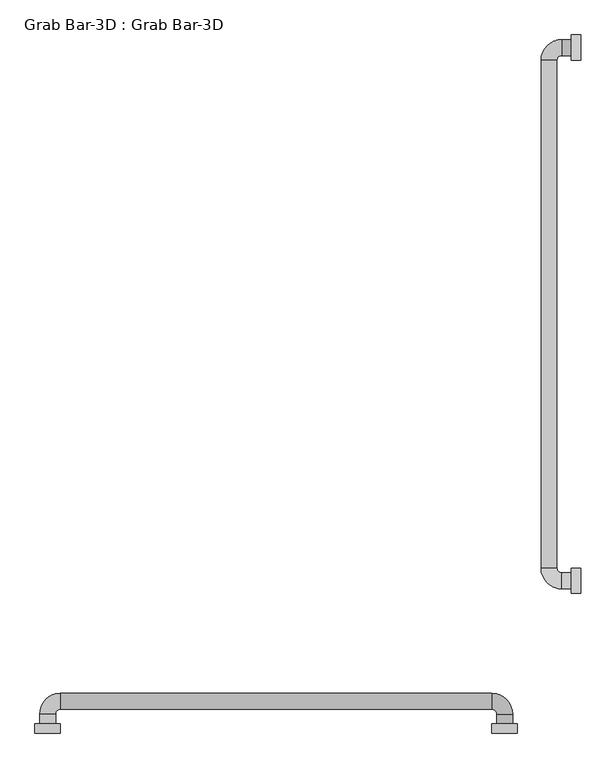
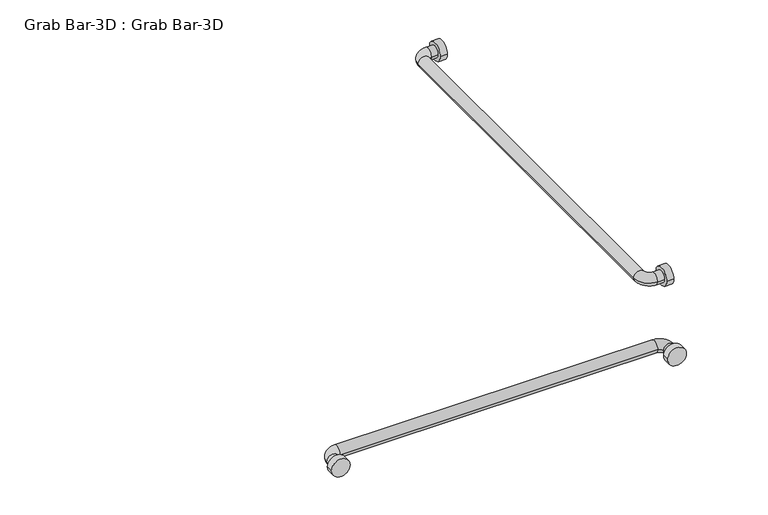
"""IFC4 building model written with IfcOpenShell, lengths in millimetres: proxy geometry, Grab Bar-3D : Grab Bar-3D."""

import ifcopenshell
import ifcopenshell.guid

model = None  # the IFC model being written
_history = None  # IfcOwnerHistory: only IFC2X3 demands one
_inside = {}  # id of a spatial element -> (the spatial element, [elements in it])
_under = {}  # id of a project, library or spatial element -> (it, [spatial elements below it])
_declared = {}  # id of a project -> (the project, [libraries it declares])
_typed = {}  # id of a type object -> (the type object, [elements of that type])
_made_of = {}  # id of a material, layer set ... -> (it, [elements and type objects made of it])


def new_model(schema):
    """Start an empty IFC model of exactly this schema.

    Asked for "IFC4X3", IfcOpenShell would pick the latest addendum, in which some entities
    have other attributes; the version numbers below select the first issue.
    IFC2X3 requires an IfcOwnerHistory on every rooted entity: one is made here for all.
    """
    global model, _history
    if schema == "IFC4X3":
        model = ifcopenshell.file(schema_version=(4, 3, 0, 0))
    else:
        model = ifcopenshell.file(schema=schema)
    _inside.clear()
    _under.clear()
    _declared.clear()
    _typed.clear()
    _made_of.clear()
    _history = None
    if model.schema == "IFC2X3":
        org = make("IfcOrganization", Name="unknown")
        user = make(
            "IfcPersonAndOrganization",
            ThePerson=make("IfcPerson", FamilyName="unknown"),
            TheOrganization=org,
        )
        app = make(
            "IfcApplication",
            ApplicationDeveloper=org,
            Version="unknown",
            ApplicationFullName="unknown",
            ApplicationIdentifier="unknown",
        )
        _history = make(
            "IfcOwnerHistory",
            OwningUser=user,
            OwningApplication=app,
            ChangeAction="ADDED",
            CreationDate=0,
        )
    return model


def make(cls, **values):
    """One entity of the class cls with the attributes given. An attribute that is None is left unset."""
    return model.create_entity(
        cls, **{name: value for name, value in values.items() if value is not None}
    )


def rooted(cls, **values):
    """An entity with a GlobalId (a new one), such as an element, a storey or a relation."""
    return make(cls, GlobalId=ifcopenshell.guid.new(), OwnerHistory=_history, **values)


def si_unit(unit_type, name, prefix=None):
    """IfcSIUnit, for example si_unit("LENGTHUNIT", "METRE", prefix="MILLI")."""
    return make("IfcSIUnit", UnitType=unit_type, Prefix=prefix, Name=name)


def assignment(units):
    """IfcUnitAssignment: the units of a project."""
    return None if units is None else make("IfcUnitAssignment", Units=units)


def point(xyz):
    """IfcCartesianPoint."""
    return None if xyz is None else make("IfcCartesianPoint", Coordinates=xyz)


def direction(xyz):
    """IfcDirection."""
    return None if xyz is None else make("IfcDirection", DirectionRatios=xyz)


def frame(location, z_axis=None, x_axis=None):
    """IfcAxis2Placement3D, a coordinate frame: its origin and axes. An axis left out is left unset."""
    return make(
        "IfcAxis2Placement3D",
        Location=point(location),
        Axis=direction(z_axis),
        RefDirection=direction(x_axis),
    )


def frame_2d(location, x_axis=None):
    """IfcAxis2Placement2D, a coordinate frame in the plane: its origin and x axis."""
    return make(
        "IfcAxis2Placement2D", Location=point(location), RefDirection=direction(x_axis)
    )


def origin():
    """The frame at (0, 0, 0) with its axes left unset."""
    return frame((0.0, 0.0, 0.0))


def place(relative_to, where):
    """IfcLocalPlacement: puts the frame where relative to a parent placement (None: the world)."""
    return make(
        "IfcLocalPlacement", PlacementRelTo=relative_to, RelativePlacement=where
    )


def context(
    kind, dimensions, precision=None, world=None, true_north=None, identifier=None
):
    """IfcGeometricRepresentationContext, for example the 3D "Model" context."""
    return make(
        "IfcGeometricRepresentationContext",
        ContextIdentifier=identifier,
        ContextType=kind,
        CoordinateSpaceDimension=dimensions,
        Precision=precision,
        WorldCoordinateSystem=world,
        TrueNorth=true_north,
    )


def project(units=None, contexts=None):
    """IfcProject with its units and contexts."""
    return rooted(
        "IfcProject",
        Name="project",
        RepresentationContexts=contexts,
        UnitsInContext=assignment(units),
    )


def spatial(cls, under=None, at=None, **own):
    """A site, building, storey or space (cls), placed at a placement, below another one or the project."""
    s = rooted(cls, ObjectPlacement=at, **own)
    if under is not None:
        _under.setdefault(under.id(), (under, []))[1].append(s)
    return s


def circle_curve(where, radius):
    """IfcCircle in the frame where."""
    return make("IfcCircle", Position=where, Radius=radius)


def ellipse_curve(where, semi_axis1, semi_axis2):
    """IfcEllipse in the frame where."""
    return make(
        "IfcEllipse", Position=where, SemiAxis1=semi_axis1, SemiAxis2=semi_axis2
    )


def trimmed(basis, trim1, trim2, sense, master):
    """IfcTrimmedCurve: the piece of a basis curve between two trims."""
    return make(
        "IfcTrimmedCurve",
        BasisCurve=basis,
        Trim1=trim1,
        Trim2=trim2,
        SenseAgreement=sense,
        MasterRepresentation=master,
    )


def segment(curve, same_sense, transition):
    """IfcCompositeCurveSegment."""
    return make(
        "IfcCompositeCurveSegment",
        Transition=transition,
        SameSense=same_sense,
        ParentCurve=curve,
    )


def composite_curve(segments, self_intersect=None):
    """IfcCompositeCurve: segments joined end to end."""
    return make("IfcCompositeCurve", Segments=segments, SelfIntersect=self_intersect)


def outline(outer, holes=None, kind="AREA"):
    """IfcArbitraryClosedProfileDef: a profile drawn as a closed curve; with holes, ...WithVoids."""
    if holes is None:
        return make("IfcArbitraryClosedProfileDef", ProfileType=kind, OuterCurve=outer)
    return make(
        "IfcArbitraryProfileDefWithVoids",
        ProfileType=kind,
        OuterCurve=outer,
        InnerCurves=holes,
    )


def extrude(swept, where, along, depth):
    """IfcExtrudedAreaSolid: the profile swept, set in the frame where, extruded along a direction by depth."""
    return make(
        "IfcExtrudedAreaSolid",
        SweptArea=swept,
        Position=where,
        ExtrudedDirection=direction(along),
        Depth=depth,
    )


def shape(context_of_items, identifier, shape_type, items):
    """IfcShapeRepresentation: the items that make up one representation, for example the "Body"."""
    return make(
        "IfcShapeRepresentation",
        ContextOfItems=context_of_items,
        RepresentationIdentifier=identifier,
        RepresentationType=shape_type,
        Items=items,
    )


def source(mapping_origin, context_of_items, identifier, shape_type, items):
    """IfcRepresentationMap: a shape defined once, which mapped items show again and again."""
    return make(
        "IfcRepresentationMap",
        MappingOrigin=mapping_origin,
        MappedRepresentation=shape(context_of_items, identifier, shape_type, items),
    )


def transform(
    local_origin,
    x_axis=None,
    y_axis=None,
    z_axis=None,
    scale=None,
    scale2=None,
    scale3=None,
    uniform=True,
):
    """IfcCartesianTransformationOperator3D, or its non-uniform kind. x_axis, y_axis, z_axis: its Axis1, 2, 3."""
    if uniform:
        return make(
            "IfcCartesianTransformationOperator3D",
            Axis1=direction(x_axis),
            Axis2=direction(y_axis),
            LocalOrigin=point(local_origin),
            Scale=scale,
            Axis3=direction(z_axis),
        )
    return make(
        "IfcCartesianTransformationOperator3DnonUniform",
        Axis1=direction(x_axis),
        Axis2=direction(y_axis),
        LocalOrigin=point(local_origin),
        Scale=scale,
        Axis3=direction(z_axis),
        Scale2=scale2,
        Scale3=scale3,
    )


def mapped(mapping_source, mapping_target):
    """IfcMappedItem: shows the shape of a source again, moved by a transform."""
    return make(
        "IfcMappedItem", MappingSource=mapping_source, MappingTarget=mapping_target
    )


def made_of(thing, what):
    """Note that an element or type object is made of a material, layer set ...; save() writes the relation."""
    if what is not None:
        _made_of.setdefault(what.id(), (what, []))[1].append(thing)
    return thing


def element(
    cls,
    number,
    at=None,
    inside=None,
    cuts=None,
    type_object=None,
    material=None,
    context=None,
    identifier="Body",
    shape_type=None,
    held_by="IfcProductDefinitionShape",
    body=None,
    shapes=None,
    **own,
):
    """One element of the class cls, such as IfcWall. Its Tag is "e" and its number.

    at: its placement. inside: the storey or other place that contains it. cuts: it is an
    opening in that element (IfcRelVoidsElement). A single representation is given by context,
    identifier, shape_type and body (its items); several are given by shapes. held_by: the class
    of the entity that holds the representations. save() writes the other relations.
    """
    e = rooted(cls, Tag="e%d" % number, ObjectPlacement=at, **own)
    if body is not None:
        shapes = [shape(context, identifier, shape_type, body)]
    if shapes is not None:
        e.Representation = make(held_by, Representations=shapes)
    if inside is not None:
        _inside.setdefault(inside.id(), (inside, []))[1].append(e)
    if cuts is not None:
        rooted(
            "IfcRelVoidsElement", RelatingBuildingElement=cuts, RelatedOpeningElement=e
        )
    if type_object is not None:
        _typed.setdefault(type_object.id(), (type_object, []))[1].append(e)
    return made_of(e, material)


def aggregate(whole, parts):
    """IfcRelAggregates: a whole, such as a stair, and the parts it consists of."""
    return rooted("IfcRelAggregates", RelatingObject=whole, RelatedObjects=parts)


def save(model, path):
    """Write the relations noted so far, then the file.

    IfcRelAggregates (storeys below a building ...), IfcRelContainedInSpatialStructure (elements
    in a storey), IfcRelDefinesByType, IfcRelAssociatesMaterial and IfcRelDeclares: one each for
    every whole, place, type object, material and project.
    """
    for whole, parts in _under.values():
        aggregate(whole, parts)
    for where, things in _inside.values():
        rooted(
            "IfcRelContainedInSpatialStructure",
            RelatedElements=things,
            RelatingStructure=where,
        )
    for kind, things in _typed.values():
        rooted("IfcRelDefinesByType", RelatedObjects=things, RelatingType=kind)
    for what, things in _made_of.values():
        rooted("IfcRelAssociatesMaterial", RelatedObjects=things, RelatingMaterial=what)
    for by, libraries in _declared.values():
        rooted("IfcRelDeclares", RelatingContext=by, RelatedDefinitions=libraries)
    model.write(path)


def plane_surface(at):
    """IfcPlane: the flat surface through the origin of the frame at, square to its z axis."""
    return make("IfcPlane", Position=at)


def cylinder_surface(at, radius):
    """IfcCylindricalSurface: all points at the distance radius from the z axis of the frame at."""
    return make("IfcCylindricalSurface", Position=at, Radius=radius)


def revolved_surface(curve, axis_point, axis_direction):
    """IfcSurfaceOfRevolution: the curve turned about the line through axis_point along axis_direction."""
    return make(
        "IfcSurfaceOfRevolution",
        SweptCurve=make("IfcArbitraryOpenProfileDef", ProfileType="CURVE", Curve=curve),
        AxisPosition=make("IfcAxis1Placement", Location=point(axis_point), Axis=direction(axis_direction)),
    )


def advanced_brep(points, edges, surfaces, faces):
    """IfcAdvancedBrep: a solid bounded by faces that lie on surfaces and meet in shared edges.

    An edge is (start, end): straight between two places in points (the first is 0);
    or (start, end, curve); or (start, end, curve, False) where it runs against its curve.
    A face is (place in surfaces, loops), or (place, loops, False) where it looks against
    its surface's normal. A loop lists edges by number (the first is 1), with a minus sign
    where the edge is run from its end to its start. The first loop is the outer one.
    """
    corners = [point(p) for p in points]
    vertices = [make("IfcVertexPoint", VertexGeometry=c) for c in corners]
    made = []
    for start, end, *more in edges:
        made.append(
            make(
                "IfcEdgeCurve",
                EdgeStart=vertices[start],
                EdgeEnd=vertices[end],
                EdgeGeometry=more[0] if more else make("IfcPolyline", Points=[corners[start], corners[end]]),
                SameSense=more[1] if len(more) > 1 else True,
            )
        )
    hull = []
    for where, loops, *sense in faces:
        bounds = []
        for j, loop in enumerate(loops):
            ring = [make("IfcOrientedEdge", EdgeElement=made[abs(k) - 1], Orientation=k > 0) for k in loop]
            bounds.append(
                make(
                    "IfcFaceOuterBound" if j == 0 else "IfcFaceBound",
                    Bound=make("IfcEdgeLoop", EdgeList=ring),
                    Orientation=True,
                )
            )
        hull.append(make("IfcAdvancedFace", Bounds=bounds, FaceSurface=surfaces[where], SameSense=sense[0] if sense else True))
    return make("IfcAdvancedBrep", Outer=make("IfcClosedShell", CfsFaces=hull))


def grab_bar_3d_grab_bar_3d_00f4341b(model_context):
    return source(origin(), model_context, "Body", "SolidModel", [
        extrude(outline(composite_curve([segment(trimmed(circle_curve(frame_2d((304.8, 914.4)), 25.4), [point((279.4, 914.4))], [point((330.2, 914.4))], False, "CARTESIAN"), True, "CONTINUOUS"), segment(trimmed(circle_curve(frame_2d((304.8, 914.4)), 25.4), [point((330.2, 914.4))], [point((279.4, 914.4))], False, "CARTESIAN"), True, "CONTINUOUS")], self_intersect=False)), frame((-19.05, 0.0, 0.0), z_axis=(1.0, 0.0, 0.0), x_axis=(0.0, 1.0, 0.0)), (0.0, 0.0, 1.0), 19.05),
        extrude(outline(composite_curve([segment(trimmed(circle_curve(frame_2d((1371.6, 914.4)), 25.4), [point((1346.2, 914.4))], [point((1397.0, 914.4))], False, "CARTESIAN"), True, "CONTINUOUS"), segment(trimmed(circle_curve(frame_2d((1371.6, 914.4)), 25.4), [point((1397.0, 914.4))], [point((1346.2, 914.4))], False, "CARTESIAN"), True, "CONTINUOUS")], self_intersect=False)), frame((-19.05, 0.0, 0.0), z_axis=(1.0, 0.0, 0.0), x_axis=(0.0, 1.0, 0.0)), (0.0, 0.0, 1.0), 19.05),
        extrude(outline(composite_curve([segment(trimmed(circle_curve(frame_2d((914.4, -152.4)), 25.4), [point((914.4, -177.8))], [point((914.4, -127.0))], False, "CARTESIAN"), True, "CONTINUOUS"), segment(trimmed(circle_curve(frame_2d((914.4, -152.4)), 25.4), [point((914.4, -127.0))], [point((914.4, -177.8))], False, "CARTESIAN"), True, "CONTINUOUS")], self_intersect=False)), frame((0.0, 0.0, 0.0), z_axis=(0.0, 1.0, 0.0), x_axis=(0.0, 0.0, 1.0)), (0.0, 0.0, 1.0), 19.05),
        extrude(outline(composite_curve([segment(trimmed(circle_curve(frame_2d((914.4, -1066.8)), 25.4), [point((914.4, -1092.2))], [point((914.4, -1041.4))], False, "CARTESIAN"), True, "CONTINUOUS"), segment(trimmed(circle_curve(frame_2d((914.4, -1066.8)), 25.4), [point((914.4, -1041.4))], [point((914.4, -1092.2))], False, "CARTESIAN"), True, "CONTINUOUS")], self_intersect=False)), frame((0.0, 0.0, 0.0), z_axis=(0.0, 1.0, 0.0), x_axis=(0.0, 0.0, 1.0)), (0.0, 0.0, 1.0), 19.05),
        advanced_brep(
        [(-19.05, 320.675, 914.4), (-19.05, 288.925, 914.4), (-38.1, 320.675, 914.4), (-38.1, 288.925, 914.4), (-79.375, 330.2, 914.4), (-47.625, 330.2, 914.4), (-47.625, 1346.2, 914.4), (-79.375, 1346.2, 914.4), (-38.1, 1387.475, 914.4), (-38.1, 1355.725, 914.4), (-19.05, 1355.725, 914.4), (-19.05, 1387.475, 914.4)],
        [
            (0, 1, circle_curve(frame((-19.05, 304.8, 914.4), z_axis=(1.0, 0.0, 0.0), x_axis=(0.0, -1.0, 0.0)), 15.875)),
            (1, 0, circle_curve(frame((-19.05, 304.8, 914.4), z_axis=(1.0, 0.0, 0.0), x_axis=(0.0, -1.0, 0.0)), 15.875)),
            (0, 2),
            (2, 3, circle_curve(frame((-38.1, 304.8, 914.4), z_axis=(1.0, 0.0, 0.0), x_axis=(0.0, -1.0, 0.0)), 15.875)),
            (3, 1),
            (3, 2, circle_curve(frame((-38.1, 304.8, 914.4), z_axis=(1.0, 0.0, 0.0), x_axis=(0.0, -1.0, 0.0)), 15.875)),
            (4, 3, circle_curve(frame((-38.1, 330.2, 914.4), z_axis=(0.0, 0.0, 1.0), x_axis=(0.0, -1.0, 0.0)), 41.275)),
            (2, 5, circle_curve(frame((-38.1, 330.2, 914.4), z_axis=(0.0, 0.0, -1.0), x_axis=(0.0, -1.0, 0.0)), 9.525)),
            (5, 4, circle_curve(frame((-63.5, 330.2, 914.4), z_axis=(0.0, -1.0, 0.0), x_axis=(-1.0, 0.0, 0.0)), 15.875)),
            (4, 5, circle_curve(frame((-63.5, 330.2, 914.4), z_axis=(0.0, -1.0, 0.0), x_axis=(-1.0, 0.0, 0.0)), 15.875)),
            (5, 6),
            (6, 7, circle_curve(frame((-63.5, 1346.2, 914.4), z_axis=(0.0, -1.0, 0.0), x_axis=(-1.0, 0.0, 0.0)), 15.875)),
            (7, 4),
            (7, 6, circle_curve(frame((-63.5, 1346.2, 914.4), z_axis=(0.0, -1.0, 0.0), x_axis=(-1.0, 0.0, 0.0)), 15.875)),
            (8, 7, circle_curve(frame((-38.1, 1346.2, 914.4), z_axis=(0.0, 0.0, 1.0), x_axis=(-1.0, 0.0, 0.0)), 41.275)),
            (6, 9, circle_curve(frame((-38.1, 1346.2, 914.4), z_axis=(0.0, 0.0, -1.0), x_axis=(-1.0, 0.0, 0.0)), 9.525)),
            (9, 8, circle_curve(frame((-38.1, 1371.6, 914.4), z_axis=(-1.0, 0.0, 0.0), x_axis=(0.0, 1.0, 0.0)), 15.875)),
            (8, 9, circle_curve(frame((-38.1, 1371.6, 914.4), z_axis=(-1.0, 0.0, 0.0), x_axis=(0.0, 1.0, 0.0)), 15.875)),
            (10, 11, circle_curve(frame((-19.05, 1371.6, 914.4), z_axis=(1.0, 0.0, 0.0), x_axis=(0.0, 1.0, 0.0)), 15.875)),
            (11, 10, circle_curve(frame((-19.05, 1371.6, 914.4), z_axis=(1.0, 0.0, 0.0), x_axis=(0.0, 1.0, 0.0)), 15.875)),
            (9, 10),
            (11, 8),
        ],
        [
            plane_surface(frame((-19.05, 304.8, -930.275), z_axis=(1.0, 0.0, 0.0), x_axis=(0.0, -1.0, 0.0))),
            cylinder_surface(frame((-19.05, 304.8, 914.4), z_axis=(1.0, 0.0, 0.0), x_axis=(0.0, -1.0, 0.0)), 15.875),
            revolved_surface(trimmed(ellipse_curve(frame((-38.1, 304.8, 914.4), z_axis=(1.0, 0.0, 0.0), x_axis=(0.0, -1.0, 0.0)), 15.875, 15.875), [point((-38.1, 320.675, 914.4))], [point((-38.1, 288.925, 914.4))], True, "CARTESIAN"), (-38.1, 330.2, 0.0), (0.0, 0.0, -1.0)),
            revolved_surface(trimmed(ellipse_curve(frame((-38.1, 304.8, 914.4), z_axis=(1.0, 0.0, 0.0), x_axis=(0.0, -1.0, 0.0)), 15.875, 15.875), [point((-38.1, 288.925, 914.4))], [point((-38.1, 320.675, 914.4))], True, "CARTESIAN"), (-38.1, 330.2, 0.0), (0.0, 0.0, -1.0)),
            cylinder_surface(frame((-63.5, 330.2, 914.4), z_axis=(0.0, -1.0, 0.0), x_axis=(-1.0, 0.0, 0.0)), 15.875),
            revolved_surface(trimmed(ellipse_curve(frame((-63.5, 1346.2, 914.4), z_axis=(0.0, -1.0, 0.0), x_axis=(-1.0, 0.0, 0.0)), 15.875, 15.875), [point((-47.625, 1346.2, 914.4))], [point((-79.375, 1346.2, 914.4))], True, "CARTESIAN"), (-38.1, 1346.2, 0.0), (0.0, 0.0, -1.0)),
            revolved_surface(trimmed(ellipse_curve(frame((-63.5, 1346.2, 914.4), z_axis=(0.0, -1.0, 0.0), x_axis=(-1.0, 0.0, 0.0)), 15.875, 15.875), [point((-79.375, 1346.2, 914.4))], [point((-47.625, 1346.2, 914.4))], True, "CARTESIAN"), (-38.1, 1346.2, 0.0), (0.0, 0.0, -1.0)),
            plane_surface(frame((-19.05, 1371.6, -930.275), z_axis=(1.0, 0.0, 0.0), x_axis=(0.0, 1.0, 0.0))),
            cylinder_surface(frame((-38.1, 1371.6, 914.4), z_axis=(-1.0, 0.0, 0.0), x_axis=(0.0, 1.0, 0.0)), 15.875),
        ],
        [
            (0, [[1, 2]]),
            (1, [[-1, 3, 4, 5]]),
            (1, [[-2, -5, 6, -3]]),
            (2, [[7, -4, 8, 9]]),
            (3, [[-8, -6, -7, 10]]),
            (4, [[-9, 11, 12, 13]]),
            (4, [[-10, -13, 14, -11]]),
            (5, [[15, -12, 16, 17]]),
            (6, [[-16, -14, -15, 18]]),
            (7, [[19, 20]]),
            (8, [[-17, 21, -20, 22]]),
            (8, [[-18, -22, -19, -21]]),
        ],
    ),
        advanced_brep(
        [(-1050.925, 19.05, 914.4), (-1082.675, 19.05, 914.4), (-1050.925, 38.1, 914.4), (-1082.675, 38.1, 914.4), (-1041.4, 79.375, 914.4), (-1041.4, 47.625, 914.4), (-177.8, 47.625, 914.4), (-177.8, 79.375, 914.4), (-136.525, 38.1, 914.4), (-168.275, 38.1, 914.4), (-168.275, 19.05, 914.4), (-136.525, 19.05, 914.4)],
        [
            (0, 1, circle_curve(frame((-1066.8, 19.05, 914.4), z_axis=(0.0, -1.0, 0.0), x_axis=(-1.0, 0.0, 0.0)), 15.875)),
            (1, 0, circle_curve(frame((-1066.8, 19.05, 914.4), z_axis=(0.0, -1.0, 0.0), x_axis=(-1.0, 0.0, 0.0)), 15.875)),
            (0, 2),
            (2, 3, circle_curve(frame((-1066.8, 38.1, 914.4), z_axis=(0.0, -1.0, 0.0), x_axis=(-1.0, 0.0, 0.0)), 15.875)),
            (3, 1),
            (3, 2, circle_curve(frame((-1066.8, 38.1, 914.4), z_axis=(0.0, -1.0, 0.0), x_axis=(-1.0, 0.0, 0.0)), 15.875)),
            (4, 3, circle_curve(frame((-1041.4, 38.1, 914.4), z_axis=(0.0, 0.0, 1.0), x_axis=(-1.0, 0.0, 0.0)), 41.275)),
            (2, 5, circle_curve(frame((-1041.4, 38.1, 914.4), z_axis=(0.0, 0.0, -1.0), x_axis=(-1.0, 0.0, 0.0)), 9.525)),
            (5, 4, circle_curve(frame((-1041.4, 63.5, 914.4), z_axis=(-1.0, 0.0, 0.0), x_axis=(0.0, 1.0, 0.0)), 15.875)),
            (4, 5, circle_curve(frame((-1041.4, 63.5, 914.4), z_axis=(-1.0, 0.0, 0.0), x_axis=(0.0, 1.0, 0.0)), 15.875)),
            (5, 6),
            (6, 7, circle_curve(frame((-177.8, 63.5, 914.4), z_axis=(-1.0, 0.0, 0.0), x_axis=(0.0, 1.0, 0.0)), 15.875)),
            (7, 4),
            (7, 6, circle_curve(frame((-177.8, 63.5, 914.4), z_axis=(-1.0, 0.0, 0.0), x_axis=(0.0, 1.0, 0.0)), 15.875)),
            (8, 7, circle_curve(frame((-177.8, 38.1, 914.4), z_axis=(0.0, 0.0, 1.0), x_axis=(0.0, 1.0, 0.0)), 41.275)),
            (6, 9, circle_curve(frame((-177.8, 38.1, 914.4), z_axis=(0.0, 0.0, -1.0), x_axis=(0.0, 1.0, 0.0)), 9.525)),
            (9, 8, circle_curve(frame((-152.4, 38.1, 914.4), z_axis=(0.0, 1.0, 0.0), x_axis=(1.0, 0.0, 0.0)), 15.875)),
            (8, 9, circle_curve(frame((-152.4, 38.1, 914.4), z_axis=(0.0, 1.0, 0.0), x_axis=(1.0, 0.0, 0.0)), 15.875)),
            (10, 11, circle_curve(frame((-152.4, 19.05, 914.4), z_axis=(0.0, -1.0, 0.0), x_axis=(1.0, 0.0, 0.0)), 15.875)),
            (11, 10, circle_curve(frame((-152.4, 19.05, 914.4), z_axis=(0.0, -1.0, 0.0), x_axis=(1.0, 0.0, 0.0)), 15.875)),
            (9, 10),
            (11, 8),
        ],
        [
            plane_surface(frame((-1997.075, 19.05, 0.0), z_axis=(0.0, -1.0, 0.0), x_axis=(0.0, 0.0, 1.0))),
            cylinder_surface(frame((-1066.8, 19.05, 914.4), z_axis=(0.0, -1.0, 0.0), x_axis=(-1.0, 0.0, 0.0)), 15.875),
            revolved_surface(trimmed(ellipse_curve(frame((-1066.8, 38.1, 914.4), z_axis=(0.0, -1.0, 0.0), x_axis=(-1.0, 0.0, 0.0)), 15.875, 15.875), [point((-1050.925, 38.1, 914.4))], [point((-1082.675, 38.1, 914.4))], True, "CARTESIAN"), (-1041.4, 38.1, 0.0), (0.0, 0.0, -1.0)),
            revolved_surface(trimmed(ellipse_curve(frame((-1066.8, 38.1, 914.4), z_axis=(0.0, -1.0, 0.0), x_axis=(-1.0, 0.0, 0.0)), 15.875, 15.875), [point((-1082.675, 38.1, 914.4))], [point((-1050.925, 38.1, 914.4))], True, "CARTESIAN"), (-1041.4, 38.1, 0.0), (0.0, 0.0, -1.0)),
            cylinder_surface(frame((-1041.4, 63.5, 914.4), z_axis=(-1.0, 0.0, 0.0), x_axis=(0.0, 1.0, 0.0)), 15.875),
            revolved_surface(trimmed(ellipse_curve(frame((-177.8, 63.5, 914.4), z_axis=(-1.0, 0.0, 0.0), x_axis=(0.0, 1.0, 0.0)), 15.875, 15.875), [point((-177.8, 47.625, 914.4))], [point((-177.8, 79.375, 914.4))], True, "CARTESIAN"), (-177.8, 38.1, 0.0), (0.0, 0.0, -1.0)),
            revolved_surface(trimmed(ellipse_curve(frame((-177.8, 63.5, 914.4), z_axis=(-1.0, 0.0, 0.0), x_axis=(0.0, 1.0, 0.0)), 15.875, 15.875), [point((-177.8, 79.375, 914.4))], [point((-177.8, 47.625, 914.4))], True, "CARTESIAN"), (-177.8, 38.1, 0.0), (0.0, 0.0, -1.0)),
            plane_surface(frame((-1082.675, 19.05, 0.0), z_axis=(0.0, -1.0, 0.0), x_axis=(0.0, 0.0, -1.0))),
            cylinder_surface(frame((-152.4, 38.1, 914.4), z_axis=(0.0, 1.0, 0.0), x_axis=(1.0, 0.0, 0.0)), 15.875),
        ],
        [
            (0, [[1, 2]]),
            (1, [[-1, 3, 4, 5]]),
            (1, [[-2, -5, 6, -3]]),
            (2, [[7, -4, 8, 9]]),
            (3, [[-8, -6, -7, 10]]),
            (4, [[-9, 11, 12, 13]]),
            (4, [[-10, -13, 14, -11]]),
            (5, [[15, -12, 16, 17]]),
            (6, [[-16, -14, -15, 18]]),
            (7, [[19, 20]]),
            (8, [[-17, 21, -20, 22]]),
            (8, [[-18, -22, -19, -21]]),
        ],
    ),
    ])


if __name__ == "__main__":
    model = new_model("IFC4")
    model_context = context("Model", 3, world=origin())
    ifc_project = project(units=[si_unit("LENGTHUNIT", "METRE", prefix="MILLI")], contexts=[model_context])
    site = spatial("IfcSite", under=ifc_project)
    building = spatial("IfcBuilding", under=site)
    placement = place(None, origin())
    grab_bar_3d_grab_bar_3d_shape = grab_bar_3d_grab_bar_3d_00f4341b(model_context)
    element("IfcBuildingElementProxy", 1, Name="Grab Bar-3D : Grab Bar-3D", ObjectType="Grab Bar-3D : Grab Bar-3D", at=placement, inside=building, context=model_context, shape_type="MappedRepresentation", body=[
        mapped(grab_bar_3d_grab_bar_3d_shape, transform((0.0, 0.0, 0.0), x_axis=(1.0, 0.0, 0.0), y_axis=(0.0, 1.0, 0.0), z_axis=(0.0, 0.0, 1.0))),
    ])
    save(model, "model.ifc")

# Revit data of these elements
# Project information
#   Organization Name = "G3B Press"
#   Organization Description = "Paul F. Aubin Cosulting Services, Inc."
#   Building Name = "Revit Essentials for Architecture"
#   Author = "Paul F. Aubin"
#   Author Website = "https://www.paulaubin.com"
#   Copyright = "Copyright © 2020 Paul F Aubin, all rights reserved"
#   Design Option = "Main Model"
#   Project Issue Date = "8/1/2020"
#   Project Status = "Design Development"
#   Client Name = "Working with Schedules, Tags and Data"
#   Project Address = "123 State ST\nSuite 301\nChicago, IL 60606"
#   Project Name = "13 Commercial"
#   Project Number = "2020.04A"
# Type "Grab Bar-3D : Grab Bar-3D"
#   Assembly Code = "C1030200"
#   Back Bar Length = 3' - 0"
#   Mounting Height = 3' - 0"
#   Side Bar Length = 3' - 6"
#   Default Elevation = 0
# Element 1 (IfcBuildingElementProxy, "Grab Bar-3D : Grab Bar-3D")
#   Materials on its faces: "Metal - Aluminum, Brushed"
# Materials
#   "Metal - Aluminum, Brushed": class "Unassigned", colour RGB 247 247 247, transparency 0
